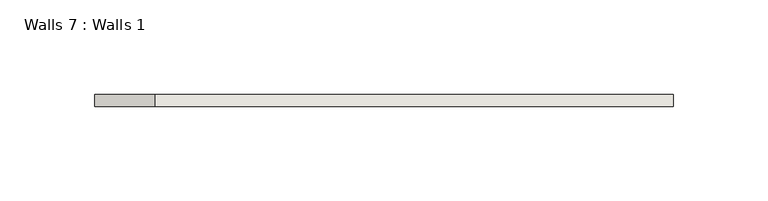
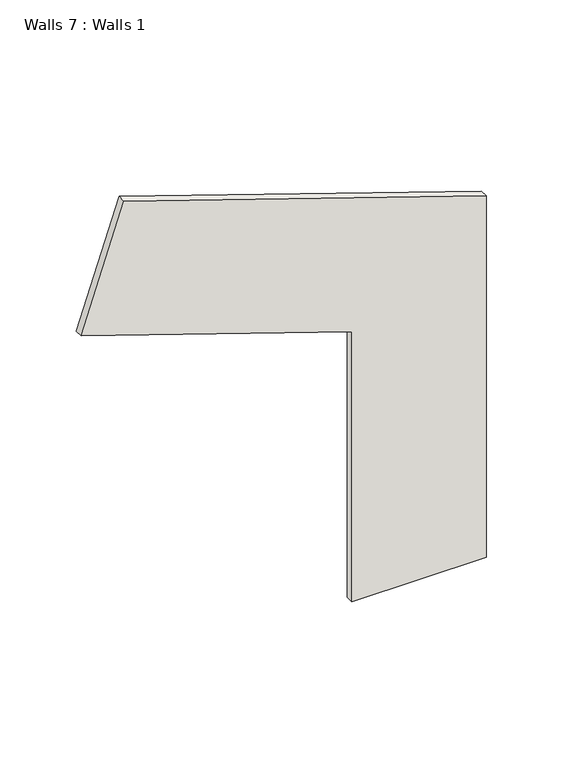
"""IFC4 building model written with IfcOpenShell, lengths in millimetres: wall geometry, Walls 7 : Walls 1."""

from ifc_helpers import new_model, si_unit, frame, origin, place, context, project, spatial, polyline, outline, extrude, source, transform, mapped, element, save


def walls_7_walls_1_756c9d08(model_context):
    return source(origin(), model_context, "Body", "SweptSolid", [
        extrude(outline(polyline([(5071.1413299, 23121.1370052), (5162.8996939, 22847.0612355), (5066.5557127, 22814.8060453), (4998.0134335, 23019.5370052), (4782.1134335, 23019.5370052), (4782.1134335, 23121.1370052), (5071.1413299, 23121.1370052)])), frame((0.0, -1122.6884634, 0.0), z_axis=(0.0, 1.0, 0.0), x_axis=(0.0, 0.0, 1.0)), (0.0, 0.0, 1.0), 6.35),
    ])


if __name__ == "__main__":
    model = new_model("IFC4")
    model_context = context("Model", 3, world=origin())
    ifc_project = project(units=[si_unit("LENGTHUNIT", "METRE", prefix="MILLI")], contexts=[model_context])
    site = spatial("IfcSite", under=ifc_project)
    building = spatial("IfcBuilding", under=site)
    placement = place(None, origin())
    walls_7_walls_1_shape = walls_7_walls_1_756c9d08(model_context)
    element("IfcWall", 1, ObjectType="Walls 7 : Walls 1", at=placement, inside=building, context=model_context, shape_type="MappedRepresentation", body=[
        mapped(walls_7_walls_1_shape, transform((0.0, 0.0, 0.0), x_axis=(1.0, 0.0, 0.0), y_axis=(0.0, 1.0, 0.0), z_axis=(0.0, 0.0, 1.0))),
    ])
    save(model, "model.ifc")

# Revit data of these elements
# Element 1 (IfcWall, "Walls 7 : Walls 1")
#   Materials on its faces: "1/4\" STEEL GUSSET PLATE - (RAW STEEL)"
# Materials
#   "1/4\" STEEL GUSSET PLATE - (RAW STEEL)": class "Metal", colour RGB 189 187 185, transparency 0, Description = "Structural steel 50ksi", Cost = 0
